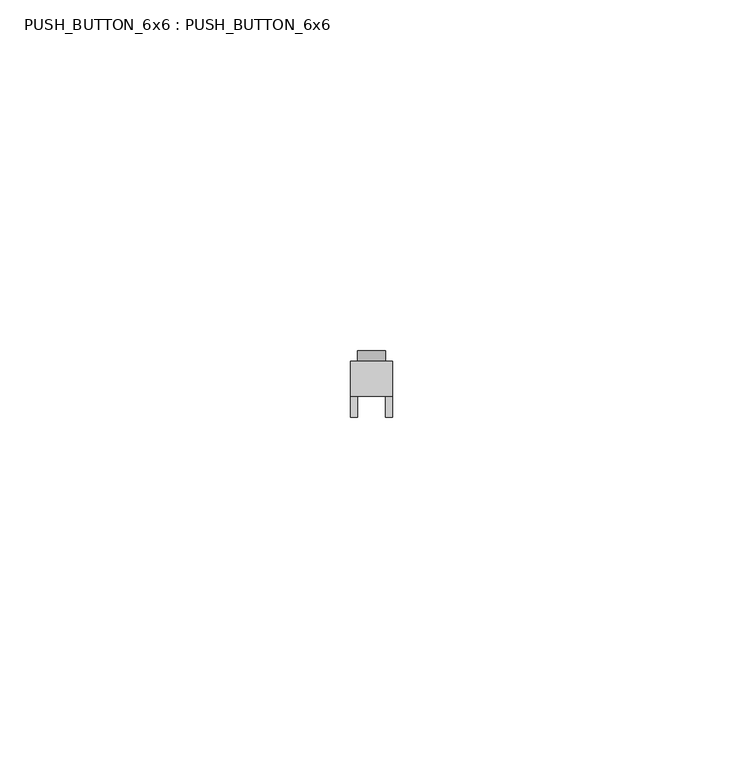
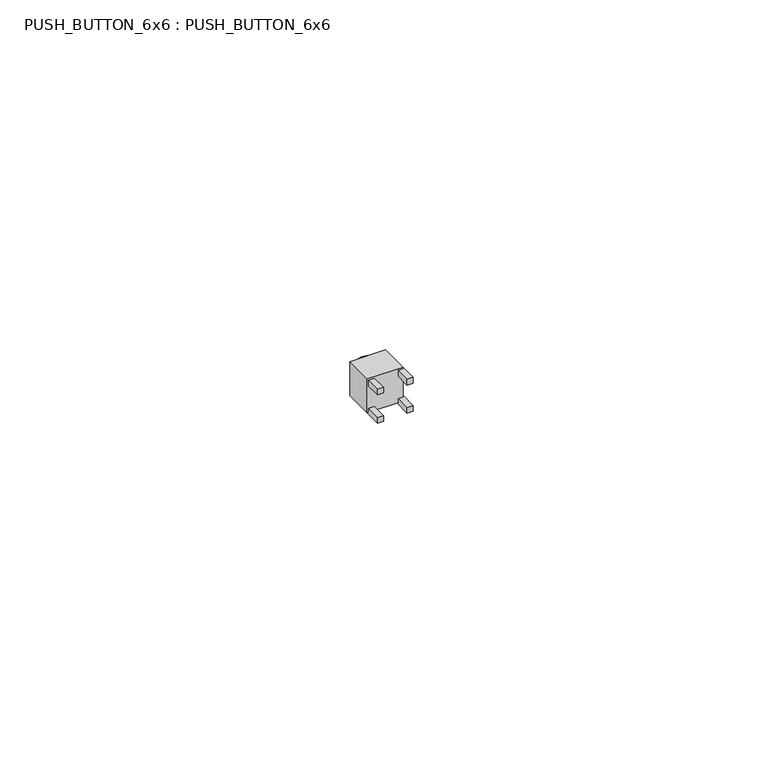
"""IFC4 building model written with IfcOpenShell, lengths in millimetres: furniture geometry, PUSH_BUTTON_6x6 : PUSH_BUTTON_6x6."""

import ifcopenshell
import ifcopenshell.guid

model = None  # the IFC model being written
_history = None  # IfcOwnerHistory: only IFC2X3 demands one
_inside = {}  # id of a spatial element -> (the spatial element, [elements in it])
_under = {}  # id of a project, library or spatial element -> (it, [spatial elements below it])
_declared = {}  # id of a project -> (the project, [libraries it declares])
_typed = {}  # id of a type object -> (the type object, [elements of that type])
_made_of = {}  # id of a material, layer set ... -> (it, [elements and type objects made of it])


def new_model(schema):
    """Start an empty IFC model of exactly this schema.

    Asked for "IFC4X3", IfcOpenShell would pick the latest addendum, in which some entities
    have other attributes; the version numbers below select the first issue.
    IFC2X3 requires an IfcOwnerHistory on every rooted entity: one is made here for all.
    """
    global model, _history
    if schema == "IFC4X3":
        model = ifcopenshell.file(schema_version=(4, 3, 0, 0))
    else:
        model = ifcopenshell.file(schema=schema)
    _inside.clear()
    _under.clear()
    _declared.clear()
    _typed.clear()
    _made_of.clear()
    _history = None
    if model.schema == "IFC2X3":
        org = make("IfcOrganization", Name="unknown")
        user = make(
            "IfcPersonAndOrganization",
            ThePerson=make("IfcPerson", FamilyName="unknown"),
            TheOrganization=org,
        )
        app = make(
            "IfcApplication",
            ApplicationDeveloper=org,
            Version="unknown",
            ApplicationFullName="unknown",
            ApplicationIdentifier="unknown",
        )
        _history = make(
            "IfcOwnerHistory",
            OwningUser=user,
            OwningApplication=app,
            ChangeAction="ADDED",
            CreationDate=0,
        )
    return model


def make(cls, **values):
    """One entity of the class cls with the attributes given. An attribute that is None is left unset."""
    return model.create_entity(
        cls, **{name: value for name, value in values.items() if value is not None}
    )


def rooted(cls, **values):
    """An entity with a GlobalId (a new one), such as an element, a storey or a relation."""
    return make(cls, GlobalId=ifcopenshell.guid.new(), OwnerHistory=_history, **values)


def si_unit(unit_type, name, prefix=None):
    """IfcSIUnit, for example si_unit("LENGTHUNIT", "METRE", prefix="MILLI")."""
    return make("IfcSIUnit", UnitType=unit_type, Prefix=prefix, Name=name)


def assignment(units):
    """IfcUnitAssignment: the units of a project."""
    return None if units is None else make("IfcUnitAssignment", Units=units)


def point(xyz):
    """IfcCartesianPoint."""
    return None if xyz is None else make("IfcCartesianPoint", Coordinates=xyz)


def direction(xyz):
    """IfcDirection."""
    return None if xyz is None else make("IfcDirection", DirectionRatios=xyz)


def frame(location, z_axis=None, x_axis=None):
    """IfcAxis2Placement3D, a coordinate frame: its origin and axes. An axis left out is left unset."""
    return make(
        "IfcAxis2Placement3D",
        Location=point(location),
        Axis=direction(z_axis),
        RefDirection=direction(x_axis),
    )


def frame_2d(location, x_axis=None):
    """IfcAxis2Placement2D, a coordinate frame in the plane: its origin and x axis."""
    return make(
        "IfcAxis2Placement2D", Location=point(location), RefDirection=direction(x_axis)
    )


def origin():
    """The frame at (0, 0, 0) with its axes left unset."""
    return frame((0.0, 0.0, 0.0))


def origin_with_axes():
    """The frame at (0, 0, 0) with the z axis (0, 0, 1) and the x axis (1, 0, 0) written out."""
    return frame((0.0, 0.0, 0.0), z_axis=(0.0, 0.0, 1.0), x_axis=(1.0, 0.0, 0.0))


def place(relative_to, where):
    """IfcLocalPlacement: puts the frame where relative to a parent placement (None: the world)."""
    return make(
        "IfcLocalPlacement", PlacementRelTo=relative_to, RelativePlacement=where
    )


def context(
    kind, dimensions, precision=None, world=None, true_north=None, identifier=None
):
    """IfcGeometricRepresentationContext, for example the 3D "Model" context."""
    return make(
        "IfcGeometricRepresentationContext",
        ContextIdentifier=identifier,
        ContextType=kind,
        CoordinateSpaceDimension=dimensions,
        Precision=precision,
        WorldCoordinateSystem=world,
        TrueNorth=true_north,
    )


def project(units=None, contexts=None):
    """IfcProject with its units and contexts."""
    return rooted(
        "IfcProject",
        Name="project",
        RepresentationContexts=contexts,
        UnitsInContext=assignment(units),
    )


def spatial(cls, under=None, at=None, **own):
    """A site, building, storey or space (cls), placed at a placement, below another one or the project."""
    s = rooted(cls, ObjectPlacement=at, **own)
    if under is not None:
        _under.setdefault(under.id(), (under, []))[1].append(s)
    return s


def polyline(points):
    """IfcPolyline through the points."""
    return make("IfcPolyline", Points=[point(p) for p in points])


def circle_curve(where, radius):
    """IfcCircle in the frame where."""
    return make("IfcCircle", Position=where, Radius=radius)


def trimmed(basis, trim1, trim2, sense, master):
    """IfcTrimmedCurve: the piece of a basis curve between two trims."""
    return make(
        "IfcTrimmedCurve",
        BasisCurve=basis,
        Trim1=trim1,
        Trim2=trim2,
        SenseAgreement=sense,
        MasterRepresentation=master,
    )


def segment(curve, same_sense, transition):
    """IfcCompositeCurveSegment."""
    return make(
        "IfcCompositeCurveSegment",
        Transition=transition,
        SameSense=same_sense,
        ParentCurve=curve,
    )


def composite_curve(segments, self_intersect=None):
    """IfcCompositeCurve: segments joined end to end."""
    return make("IfcCompositeCurve", Segments=segments, SelfIntersect=self_intersect)


def outline(outer, holes=None, kind="AREA"):
    """IfcArbitraryClosedProfileDef: a profile drawn as a closed curve; with holes, ...WithVoids."""
    if holes is None:
        return make("IfcArbitraryClosedProfileDef", ProfileType=kind, OuterCurve=outer)
    return make(
        "IfcArbitraryProfileDefWithVoids",
        ProfileType=kind,
        OuterCurve=outer,
        InnerCurves=holes,
    )


def extrude(swept, where, along, depth):
    """IfcExtrudedAreaSolid: the profile swept, set in the frame where, extruded along a direction by depth."""
    return make(
        "IfcExtrudedAreaSolid",
        SweptArea=swept,
        Position=where,
        ExtrudedDirection=direction(along),
        Depth=depth,
    )


def shape(context_of_items, identifier, shape_type, items):
    """IfcShapeRepresentation: the items that make up one representation, for example the "Body"."""
    return make(
        "IfcShapeRepresentation",
        ContextOfItems=context_of_items,
        RepresentationIdentifier=identifier,
        RepresentationType=shape_type,
        Items=items,
    )


def source(mapping_origin, context_of_items, identifier, shape_type, items):
    """IfcRepresentationMap: a shape defined once, which mapped items show again and again."""
    return make(
        "IfcRepresentationMap",
        MappingOrigin=mapping_origin,
        MappedRepresentation=shape(context_of_items, identifier, shape_type, items),
    )


def transform(
    local_origin,
    x_axis=None,
    y_axis=None,
    z_axis=None,
    scale=None,
    scale2=None,
    scale3=None,
    uniform=True,
):
    """IfcCartesianTransformationOperator3D, or its non-uniform kind. x_axis, y_axis, z_axis: its Axis1, 2, 3."""
    if uniform:
        return make(
            "IfcCartesianTransformationOperator3D",
            Axis1=direction(x_axis),
            Axis2=direction(y_axis),
            LocalOrigin=point(local_origin),
            Scale=scale,
            Axis3=direction(z_axis),
        )
    return make(
        "IfcCartesianTransformationOperator3DnonUniform",
        Axis1=direction(x_axis),
        Axis2=direction(y_axis),
        LocalOrigin=point(local_origin),
        Scale=scale,
        Axis3=direction(z_axis),
        Scale2=scale2,
        Scale3=scale3,
    )


def mapped(mapping_source, mapping_target):
    """IfcMappedItem: shows the shape of a source again, moved by a transform."""
    return make(
        "IfcMappedItem", MappingSource=mapping_source, MappingTarget=mapping_target
    )


def made_of(thing, what):
    """Note that an element or type object is made of a material, layer set ...; save() writes the relation."""
    if what is not None:
        _made_of.setdefault(what.id(), (what, []))[1].append(thing)
    return thing


def element(
    cls,
    number,
    at=None,
    inside=None,
    cuts=None,
    type_object=None,
    material=None,
    context=None,
    identifier="Body",
    shape_type=None,
    held_by="IfcProductDefinitionShape",
    body=None,
    shapes=None,
    **own,
):
    """One element of the class cls, such as IfcWall. Its Tag is "e" and its number.

    at: its placement. inside: the storey or other place that contains it. cuts: it is an
    opening in that element (IfcRelVoidsElement). A single representation is given by context,
    identifier, shape_type and body (its items); several are given by shapes. held_by: the class
    of the entity that holds the representations. save() writes the other relations.
    """
    e = rooted(cls, Tag="e%d" % number, ObjectPlacement=at, **own)
    if body is not None:
        shapes = [shape(context, identifier, shape_type, body)]
    if shapes is not None:
        e.Representation = make(held_by, Representations=shapes)
    if inside is not None:
        _inside.setdefault(inside.id(), (inside, []))[1].append(e)
    if cuts is not None:
        rooted(
            "IfcRelVoidsElement", RelatingBuildingElement=cuts, RelatedOpeningElement=e
        )
    if type_object is not None:
        _typed.setdefault(type_object.id(), (type_object, []))[1].append(e)
    return made_of(e, material)


def aggregate(whole, parts):
    """IfcRelAggregates: a whole, such as a stair, and the parts it consists of."""
    return rooted("IfcRelAggregates", RelatingObject=whole, RelatedObjects=parts)


def save(model, path):
    """Write the relations noted so far, then the file.

    IfcRelAggregates (storeys below a building ...), IfcRelContainedInSpatialStructure (elements
    in a storey), IfcRelDefinesByType, IfcRelAssociatesMaterial and IfcRelDeclares: one each for
    every whole, place, type object, material and project.
    """
    for whole, parts in _under.values():
        aggregate(whole, parts)
    for where, things in _inside.values():
        rooted(
            "IfcRelContainedInSpatialStructure",
            RelatedElements=things,
            RelatingStructure=where,
        )
    for kind, things in _typed.values():
        rooted("IfcRelDefinesByType", RelatedObjects=things, RelatingType=kind)
    for what, things in _made_of.values():
        rooted("IfcRelAssociatesMaterial", RelatedObjects=things, RelatingMaterial=what)
    for by, libraries in _declared.values():
        rooted("IfcRelDeclares", RelatingContext=by, RelatedDefinitions=libraries)
    model.write(path)


def push_button_6x6_push_button_6x6_05097e20(model_context):
    return source(origin(), model_context, "Body", "SweptSolid", [
        extrude(outline(polyline([(-3.0, 0.0), (3.0, 0.0), (3.0, -5.0), (-3.0, -5.0), (-3.0, 0.0)])), origin_with_axes(), (0.0, 0.0, 1.0), 6.0),
        extrude(outline(composite_curve([segment(trimmed(circle_curve(frame_2d((3.0, 0.0)), 2.0), [point((3.0, -2.0))], [point((3.0, 2.0))], False, "CARTESIAN"), True, "CONTINUOUS"), segment(trimmed(circle_curve(frame_2d((3.0, 0.0)), 2.0), [point((3.0, 2.0))], [point((3.0, -2.0))], False, "CARTESIAN"), True, "CONTINUOUS")], self_intersect=False)), frame((0.0, 0.0, 0.0), z_axis=(0.0, 1.0, 0.0), x_axis=(0.0, 0.0, 1.0)), (0.0, 0.0, 1.0), 1.5),
        extrude(outline(polyline([(3.0, -5.0), (3.0, -8.0), (2.0, -8.0), (2.0, -5.0), (3.0, -5.0)])), frame((0.0, 0.0, 5.0), z_axis=(0.0, 0.0, 1.0), x_axis=(1.0, 0.0, 0.0)), (0.0, 0.0, 1.0), 1.0),
        extrude(outline(polyline([(-2.0, -5.0), (-2.0, -8.0), (-3.0, -8.0), (-3.0, -5.0), (-2.0, -5.0)])), frame((0.0, 0.0, 5.0), z_axis=(0.0, 0.0, 1.0), x_axis=(1.0, 0.0, 0.0)), (0.0, 0.0, 1.0), 1.0),
        extrude(outline(polyline([(3.0, -5.0), (3.0, -8.0), (2.0, -8.0), (2.0, -5.0), (3.0, -5.0)])), origin_with_axes(), (0.0, 0.0, 1.0), 1.0),
        extrude(outline(polyline([(-2.0, -5.0), (-2.0, -8.0), (-3.0, -8.0), (-3.0, -5.0), (-2.0, -5.0)])), origin_with_axes(), (0.0, 0.0, 1.0), 1.0),
    ])


if __name__ == "__main__":
    model = new_model("IFC4")
    model_context = context("Model", 3, world=origin())
    ifc_project = project(units=[si_unit("LENGTHUNIT", "METRE", prefix="MILLI")], contexts=[model_context])
    site = spatial("IfcSite", under=ifc_project)
    building = spatial("IfcBuilding", under=site)
    placement = place(None, origin())
    push_button_6x6_push_button_6x6_shape = push_button_6x6_push_button_6x6_05097e20(model_context)
    element("IfcFurniture", 1, ObjectType="PUSH_BUTTON_6x6 : PUSH_BUTTON_6x6", at=placement, inside=building, context=model_context, shape_type="MappedRepresentation", body=[
        mapped(push_button_6x6_push_button_6x6_shape, transform((0.0, 0.0, 0.0), x_axis=(1.0, 0.0, 0.0), y_axis=(0.0, 1.0, 0.0), z_axis=(0.0, 0.0, 1.0))),
    ])
    save(model, "model.ifc")

# Revit data of these elements
# Type "PUSH_BUTTON_6x6 : PUSH_BUTTON_6x6"
#   Default Elevation = 0
# Element 1 (IfcFurniture, "PUSH_BUTTON_6x6 : PUSH_BUTTON_6x6")
#   Materials on its faces: ".BOTAO"
# Materials
#   ".BOTAO": class "Vidro", colour RGB 0 255 255, transparency 0.75, Cost = 0
